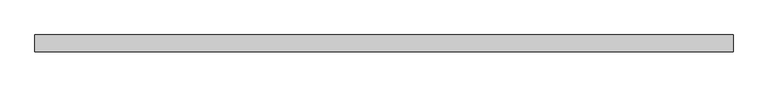
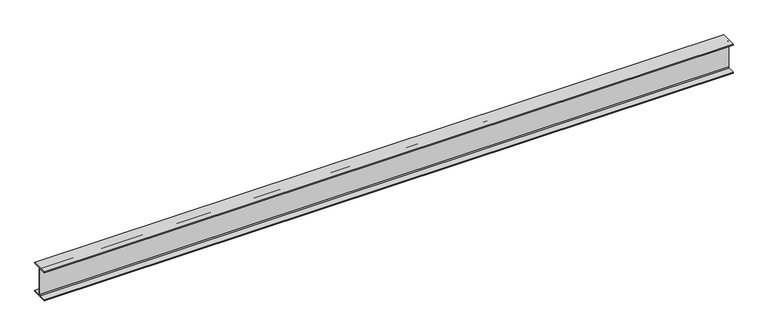
"""IFC4 building model written with IfcOpenShell, lengths in millimetres: beam geometry, Old_Steel Beam_H-KSD3502 : H_SB_ASB_H-390×300x10x16."""

from ifc_helpers import new_model, si_unit, point, frame, frame_2d, origin, place, context, project, spatial, polyline, circle_curve, trimmed, segment, composite_curve, outline, extrude, source, transform, mapped, element, save


def beam_d03452ae(model_context):
    return source(origin(), model_context, "Body", "SweptSolid", [
        extrude(outline(composite_curve([segment(polyline([(82.5, -141.5), (82.5, -151.7), (-82.5, -151.7), (-82.5, -141.5), (-11.9, -141.5)]), True, "CONTINUOUS"), segment(trimmed(circle_curve(frame_2d((-11.9, -132.6)), 8.9), [point((-11.9, -141.5))], [point((-3.0, -132.6))], True, "CARTESIAN"), True, "CONTINUOUS"), segment(polyline([(-3.0, -132.6), (-3.0, 132.6)]), True, "CONTINUOUS"), segment(trimmed(circle_curve(frame_2d((-11.9, 132.6)), 8.9), [point((-3.0, 132.6))], [point((-11.9, 141.5))], True, "CARTESIAN"), True, "CONTINUOUS"), segment(polyline([(-11.9, 141.5), (-82.5, 141.5), (-82.5, 151.7), (82.5, 151.7), (82.5, 141.5), (11.9, 141.5)]), True, "CONTINUOUS"), segment(trimmed(circle_curve(frame_2d((11.9, 132.6)), 8.9), [point((11.9, 141.5))], [point((3.0, 132.6))], True, "CARTESIAN"), True, "CONTINUOUS"), segment(polyline([(3.0, 132.6), (3.0, -132.6)]), True, "CONTINUOUS"), segment(trimmed(circle_curve(frame_2d((11.9, -132.6)), 8.9), [point((3.0, -132.6))], [point((11.9, -141.5))], True, "CARTESIAN"), True, "CONTINUOUS"), segment(polyline([(11.9, -141.5), (82.5, -141.5)]), True, "CONTINUOUS")], self_intersect=False)), frame((-3404.8, 0.0, 0.0), z_axis=(1.0, 0.0, 0.0), x_axis=(0.0, 1.0, 0.0)), (0.0, 0.0, 1.0), 6892.0999994),
    ])


if __name__ == "__main__":
    model = new_model("IFC4")
    model_context = context("Model", 3, world=origin())
    ifc_project = project(units=[si_unit("LENGTHUNIT", "METRE", prefix="MILLI")], contexts=[model_context])
    site = spatial("IfcSite", under=ifc_project)
    building = spatial("IfcBuilding", under=site)
    placement = place(None, origin())
    beam_shape = beam_d03452ae(model_context)
    element("IfcBeam", 1, ObjectType="Old_Steel Beam_H-KSD3502 : H_SB_ASB_H-390×300x10x16", at=placement, inside=building, context=model_context, shape_type="MappedRepresentation", body=[
        mapped(beam_shape, transform((0.0, 0.0, 0.0), x_axis=(1.0, 0.0, 0.0), y_axis=(0.0, 1.0, 0.0), z_axis=(0.0, 0.0, 1.0))),
    ])
    save(model, "model.ifc")

# Revit data of these elements
# Type "Old_Steel Beam_H-KSD3502 : H_SB_ASB_H-390×300x10x16"
#   Width = 30.0 cm
#   Web Thickness = 1.0 cm
#   Web Fillet = 2.2 cm
#   Warping Constant = 2517770.0 cm⁶
#   Torsional Moment of Inertia = 94.3867 cm⁴
#   Torsional Modulus = 1.0 cm³
#   Section Area = 136.0 cm²
#   Plastic Modulus weak axis = 733.0 cm³
#   Plastic Modulus strong axis = 2190.0 cm³
#   Perimeter = 1.92 m²/m
#   Nominal Weight = 107.00 kgf/m
#   Moment of Inertia weak axis = 7210.00 cm⁴
#   Moment of Inertia strong axis = 38700.00 cm⁴
#   Height = 39.0 cm
#   Flange Thickness = 1.6 cm
#   Elastic Modulus weak axis = 481.0 cm³
#   Elastic Modulus strong axis = 1980.0 cm³
#   Centroid Vertical = 19.5 cm
#   Centroid Horizontal = 15.0 cm
#   Length [instance default] = 1.5240 m
#   Structural Material [instance default] = Steel, 45-345
#   Assembly Code = ""
# Element 1 (IfcBeam, "Old_Steel Beam_H-KSD3502 : H_SB_ASB_H-390×300x10x16")
#   Structural Material = none
# Materials
#   "Steel, 45-345": class "Metal", colour RGB 189 187 185, transparency 0, Description = "Steel 345 MPa", Cost = 0
